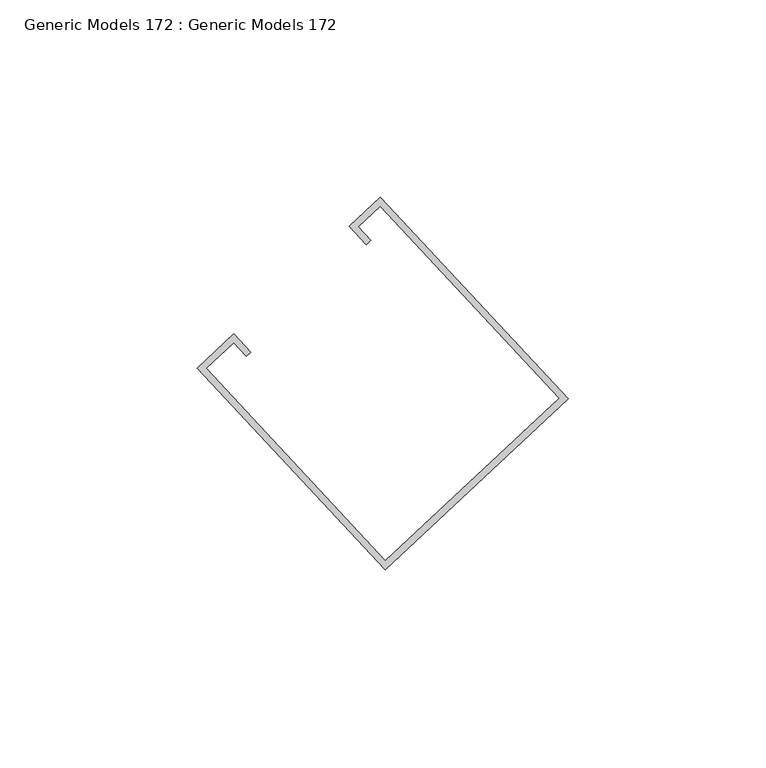
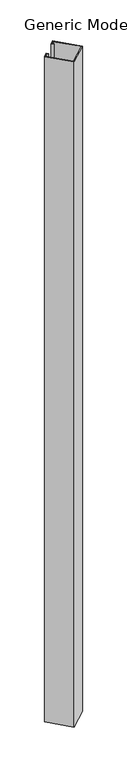
"""IFC4 building model written with IfcOpenShell, lengths in millimetres: proxy geometry, Generic Models 172 : Generic Models 172."""

import ifcopenshell
import ifcopenshell.guid

model = None  # the IFC model being written
_history = None  # IfcOwnerHistory: only IFC2X3 demands one
_inside = {}  # id of a spatial element -> (the spatial element, [elements in it])
_under = {}  # id of a project, library or spatial element -> (it, [spatial elements below it])
_declared = {}  # id of a project -> (the project, [libraries it declares])
_typed = {}  # id of a type object -> (the type object, [elements of that type])
_made_of = {}  # id of a material, layer set ... -> (it, [elements and type objects made of it])


def new_model(schema):
    """Start an empty IFC model of exactly this schema.

    Asked for "IFC4X3", IfcOpenShell would pick the latest addendum, in which some entities
    have other attributes; the version numbers below select the first issue.
    IFC2X3 requires an IfcOwnerHistory on every rooted entity: one is made here for all.
    """
    global model, _history
    if schema == "IFC4X3":
        model = ifcopenshell.file(schema_version=(4, 3, 0, 0))
    else:
        model = ifcopenshell.file(schema=schema)
    _inside.clear()
    _under.clear()
    _declared.clear()
    _typed.clear()
    _made_of.clear()
    _history = None
    if model.schema == "IFC2X3":
        org = make("IfcOrganization", Name="unknown")
        user = make(
            "IfcPersonAndOrganization",
            ThePerson=make("IfcPerson", FamilyName="unknown"),
            TheOrganization=org,
        )
        app = make(
            "IfcApplication",
            ApplicationDeveloper=org,
            Version="unknown",
            ApplicationFullName="unknown",
            ApplicationIdentifier="unknown",
        )
        _history = make(
            "IfcOwnerHistory",
            OwningUser=user,
            OwningApplication=app,
            ChangeAction="ADDED",
            CreationDate=0,
        )
    return model


def make(cls, **values):
    """One entity of the class cls with the attributes given. An attribute that is None is left unset."""
    return model.create_entity(
        cls, **{name: value for name, value in values.items() if value is not None}
    )


def rooted(cls, **values):
    """An entity with a GlobalId (a new one), such as an element, a storey or a relation."""
    return make(cls, GlobalId=ifcopenshell.guid.new(), OwnerHistory=_history, **values)


def si_unit(unit_type, name, prefix=None):
    """IfcSIUnit, for example si_unit("LENGTHUNIT", "METRE", prefix="MILLI")."""
    return make("IfcSIUnit", UnitType=unit_type, Prefix=prefix, Name=name)


def assignment(units):
    """IfcUnitAssignment: the units of a project."""
    return None if units is None else make("IfcUnitAssignment", Units=units)


def point(xyz):
    """IfcCartesianPoint."""
    return None if xyz is None else make("IfcCartesianPoint", Coordinates=xyz)


def direction(xyz):
    """IfcDirection."""
    return None if xyz is None else make("IfcDirection", DirectionRatios=xyz)


def frame(location, z_axis=None, x_axis=None):
    """IfcAxis2Placement3D, a coordinate frame: its origin and axes. An axis left out is left unset."""
    return make(
        "IfcAxis2Placement3D",
        Location=point(location),
        Axis=direction(z_axis),
        RefDirection=direction(x_axis),
    )


def origin():
    """The frame at (0, 0, 0) with its axes left unset."""
    return frame((0.0, 0.0, 0.0))


def place(relative_to, where):
    """IfcLocalPlacement: puts the frame where relative to a parent placement (None: the world)."""
    return make(
        "IfcLocalPlacement", PlacementRelTo=relative_to, RelativePlacement=where
    )


def context(
    kind, dimensions, precision=None, world=None, true_north=None, identifier=None
):
    """IfcGeometricRepresentationContext, for example the 3D "Model" context."""
    return make(
        "IfcGeometricRepresentationContext",
        ContextIdentifier=identifier,
        ContextType=kind,
        CoordinateSpaceDimension=dimensions,
        Precision=precision,
        WorldCoordinateSystem=world,
        TrueNorth=true_north,
    )


def project(units=None, contexts=None):
    """IfcProject with its units and contexts."""
    return rooted(
        "IfcProject",
        Name="project",
        RepresentationContexts=contexts,
        UnitsInContext=assignment(units),
    )


def spatial(cls, under=None, at=None, **own):
    """A site, building, storey or space (cls), placed at a placement, below another one or the project."""
    s = rooted(cls, ObjectPlacement=at, **own)
    if under is not None:
        _under.setdefault(under.id(), (under, []))[1].append(s)
    return s


def polyline(points):
    """IfcPolyline through the points."""
    return make("IfcPolyline", Points=[point(p) for p in points])


def outline(outer, holes=None, kind="AREA"):
    """IfcArbitraryClosedProfileDef: a profile drawn as a closed curve; with holes, ...WithVoids."""
    if holes is None:
        return make("IfcArbitraryClosedProfileDef", ProfileType=kind, OuterCurve=outer)
    return make(
        "IfcArbitraryProfileDefWithVoids",
        ProfileType=kind,
        OuterCurve=outer,
        InnerCurves=holes,
    )


def extrude(swept, where, along, depth):
    """IfcExtrudedAreaSolid: the profile swept, set in the frame where, extruded along a direction by depth."""
    return make(
        "IfcExtrudedAreaSolid",
        SweptArea=swept,
        Position=where,
        ExtrudedDirection=direction(along),
        Depth=depth,
    )


def shape(context_of_items, identifier, shape_type, items):
    """IfcShapeRepresentation: the items that make up one representation, for example the "Body"."""
    return make(
        "IfcShapeRepresentation",
        ContextOfItems=context_of_items,
        RepresentationIdentifier=identifier,
        RepresentationType=shape_type,
        Items=items,
    )


def source(mapping_origin, context_of_items, identifier, shape_type, items):
    """IfcRepresentationMap: a shape defined once, which mapped items show again and again."""
    return make(
        "IfcRepresentationMap",
        MappingOrigin=mapping_origin,
        MappedRepresentation=shape(context_of_items, identifier, shape_type, items),
    )


def transform(
    local_origin,
    x_axis=None,
    y_axis=None,
    z_axis=None,
    scale=None,
    scale2=None,
    scale3=None,
    uniform=True,
):
    """IfcCartesianTransformationOperator3D, or its non-uniform kind. x_axis, y_axis, z_axis: its Axis1, 2, 3."""
    if uniform:
        return make(
            "IfcCartesianTransformationOperator3D",
            Axis1=direction(x_axis),
            Axis2=direction(y_axis),
            LocalOrigin=point(local_origin),
            Scale=scale,
            Axis3=direction(z_axis),
        )
    return make(
        "IfcCartesianTransformationOperator3DnonUniform",
        Axis1=direction(x_axis),
        Axis2=direction(y_axis),
        LocalOrigin=point(local_origin),
        Scale=scale,
        Axis3=direction(z_axis),
        Scale2=scale2,
        Scale3=scale3,
    )


def mapped(mapping_source, mapping_target):
    """IfcMappedItem: shows the shape of a source again, moved by a transform."""
    return make(
        "IfcMappedItem", MappingSource=mapping_source, MappingTarget=mapping_target
    )


def made_of(thing, what):
    """Note that an element or type object is made of a material, layer set ...; save() writes the relation."""
    if what is not None:
        _made_of.setdefault(what.id(), (what, []))[1].append(thing)
    return thing


def element(
    cls,
    number,
    at=None,
    inside=None,
    cuts=None,
    type_object=None,
    material=None,
    context=None,
    identifier="Body",
    shape_type=None,
    held_by="IfcProductDefinitionShape",
    body=None,
    shapes=None,
    **own,
):
    """One element of the class cls, such as IfcWall. Its Tag is "e" and its number.

    at: its placement. inside: the storey or other place that contains it. cuts: it is an
    opening in that element (IfcRelVoidsElement). A single representation is given by context,
    identifier, shape_type and body (its items); several are given by shapes. held_by: the class
    of the entity that holds the representations. save() writes the other relations.
    """
    e = rooted(cls, Tag="e%d" % number, ObjectPlacement=at, **own)
    if body is not None:
        shapes = [shape(context, identifier, shape_type, body)]
    if shapes is not None:
        e.Representation = make(held_by, Representations=shapes)
    if inside is not None:
        _inside.setdefault(inside.id(), (inside, []))[1].append(e)
    if cuts is not None:
        rooted(
            "IfcRelVoidsElement", RelatingBuildingElement=cuts, RelatedOpeningElement=e
        )
    if type_object is not None:
        _typed.setdefault(type_object.id(), (type_object, []))[1].append(e)
    return made_of(e, material)


def aggregate(whole, parts):
    """IfcRelAggregates: a whole, such as a stair, and the parts it consists of."""
    return rooted("IfcRelAggregates", RelatingObject=whole, RelatedObjects=parts)


def save(model, path):
    """Write the relations noted so far, then the file.

    IfcRelAggregates (storeys below a building ...), IfcRelContainedInSpatialStructure (elements
    in a storey), IfcRelDefinesByType, IfcRelAssociatesMaterial and IfcRelDeclares: one each for
    every whole, place, type object, material and project.
    """
    for whole, parts in _under.values():
        aggregate(whole, parts)
    for where, things in _inside.values():
        rooted(
            "IfcRelContainedInSpatialStructure",
            RelatedElements=things,
            RelatingStructure=where,
        )
    for kind, things in _typed.values():
        rooted("IfcRelDefinesByType", RelatedObjects=things, RelatingType=kind)
    for what, things in _made_of.values():
        rooted("IfcRelAssociatesMaterial", RelatedObjects=things, RelatingMaterial=what)
    for by, libraries in _declared.values():
        rooted("IfcRelDeclares", RelatingContext=by, RelatedDefinitions=libraries)
    model.write(path)


def generic_models_172_generic_models_172_0ce5b567(model_context):
    return source(origin(), model_context, "Body", "SweptSolid", [
        extrude(outline(polyline([(-438.6289329, -19897.2170189), (-445.5950769, -19903.7130533), (-400.1228362, -19952.4760614), (-356.0039242, -19911.3345103), (-401.4761648, -19862.5715022), (-407.0527368, -19867.7717397), (-403.8047196, -19871.2548117), (-404.9657436, -19872.3374841), (-409.2964332, -19867.6933881), (-401.3978132, -19860.3278058), (-353.7602278, -19911.4128619), (-400.2011878, -19954.7197578), (-447.8387733, -19903.6347017), (-438.5505813, -19894.9733225), (-434.2198917, -19899.6174185), (-435.3809157, -19900.7000909), (-438.6289329, -19897.2170189)])), frame((0.0, 0.0, 831.85), z_axis=(0.0, 0.0, 1.0), x_axis=(1.0, 0.0, 0.0)), (0.0, 0.0, 1.0), 1822.45),
    ])


if __name__ == "__main__":
    model = new_model("IFC4")
    model_context = context("Model", 3, world=origin())
    ifc_project = project(units=[si_unit("LENGTHUNIT", "METRE", prefix="MILLI")], contexts=[model_context])
    site = spatial("IfcSite", under=ifc_project)
    building = spatial("IfcBuilding", under=site)
    placement = place(None, origin())
    generic_models_172_generic_models_172_shape = generic_models_172_generic_models_172_0ce5b567(model_context)
    element("IfcBuildingElementProxy", 1, Name="Generic Models 172 : Generic Models 172", ObjectType="Generic Models 172 : Generic Models 172", at=placement, inside=building, context=model_context, shape_type="MappedRepresentation", body=[
        mapped(generic_models_172_generic_models_172_shape, transform((0.0, 0.0, 0.0), x_axis=(1.0, 0.0, 0.0), y_axis=(0.0, 1.0, 0.0), z_axis=(0.0, 0.0, 1.0))),
    ])
    save(model, "model.ifc")

# Revit data of these elements
# Element 1 (IfcBuildingElementProxy, "Generic Models 172 : Generic Models 172")
#   Materials on its faces: "GALVANIZED UNISTRUT P5500, 1 5/8\" X 2 7/16\" OR ALUM. CHANNEL"
# Materials
#   "GALVANIZED UNISTRUT P5500, 1 5/8\" X 2 7/16\" OR ALUM. CHANNEL": class "Metal", colour RGB 244 244 244, transparency 0, Description = "Aluminum 6061", Cost = 0
